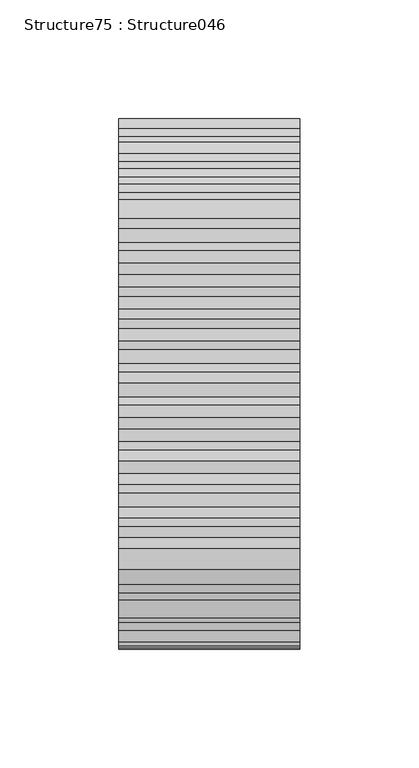
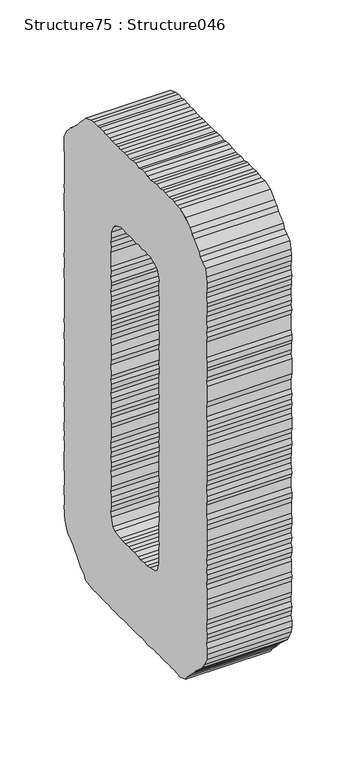
"""IFC4 building model written with IfcOpenShell, lengths in millimetres: proxy geometry, Structure75 : Structure046."""

from ifc_helpers import new_model, si_unit, frame, origin, place, context, project, spatial, polyline, outline, extrude, source, transform, mapped, element, save


def structure75_structure046_599be4c7(model_context):
    return source(origin(), model_context, "Body", "SweptSolid", [
        extrude(outline(polyline([(278111.8907934, 3554.0087015), (278103.1103976, 3552.242032), (278099.0090285, 3551.6675836), (278094.9092641, 3552.242032), (278090.2286327, 3552.242032), (278084.9478793, 3551.6675836), (278080.267248, 3551.6675836), (278076.1658789, 3552.242032), (278070.8851255, 3551.0658569), (278065.625232, 3551.6675836), (278061.5013985, 3551.0658569), (278057.401634, 3551.0658569), (278052.7210027, 3552.242032), (278048.0195115, 3552.242032), (278043.3613446, 3551.6675836), (278029.2761264, 3551.6675836), (278024.0162328, 3552.242032), (278019.9164683, 3552.242032), (278015.2133726, 3551.0658569), (278010.5343459, 3551.0658569), (278006.4329768, 3552.242032), (278001.1506188, 3551.6675836), (277997.652581, 3552.242032), (277991.7909607, 3551.6675836), (277987.6687318, 3551.6675836), (277982.4088383, 3552.242032), (277978.3074692, 3551.6675836), (277974.2077047, 3552.242032), (277969.5270734, 3551.6675836), (277964.2447154, 3551.0658569), (277956.0435818, 3554.0087015), (277953.1248062, 3558.1100706), (277946.6614593, 3564.54293), (277943.7426837, 3568.0682461), (277939.6413146, 3572.1423369), (277936.1208124, 3575.0851816), (277933.2004322, 3578.0103756), (277929.6799299, 3580.9532202), (277926.7595497, 3585.6274331), (277923.2390475, 3592.6700423), (277922.6373208, 3597.9540049), (277922.6373208, 3603.2122938), (277923.8183097, 3607.8961343), (277923.2390475, 3612.5976255), (277922.6373208, 3616.69739), (277923.8183097, 3621.3732075), (277923.8183097, 3625.472972), (277923.2390475, 3630.1824862), (277923.2390475, 3640.7167147), (277922.6373208, 3645.4262289), (277923.2390475, 3649.5003197), (277923.2390475, 3659.4584952), (277923.8183097, 3663.5598643), (277922.6373208, 3668.8261762), (277922.6373208, 3673.5276674), (277923.8183097, 3677.0449605), (277922.6373208, 3682.3289231), (277923.8183097, 3686.4030139), (277923.2390475, 3691.6869765), (277922.6373208, 3696.3884676), (277922.6373208, 3701.0723082), (277923.2390475, 3705.1720727), (277923.2390475, 3715.7143242), (277922.6373208, 3720.9726131), (277922.6373208, 3725.0996559), (277923.8183097, 3730.3563402), (277923.8183097, 3739.1592005), (277922.6373208, 3743.2332913), (277923.2390475, 3747.9428055), (277923.8183097, 3753.2171405), (277923.8183097, 3757.8753073), (277923.2390475, 3762.5848215), (277923.2390475, 3767.2590344), (277922.6373208, 3771.3860772), (277923.2390475, 3777.2444882), (277923.2390475, 3781.9299333), (277922.6373208, 3786.6298199), (277922.6373208, 3795.960595), (277923.2390475, 3800.6717138), (277923.2390475, 3805.3459267), (277922.6373208, 3810.0474179), (277923.2390475, 3813.5743386), (277922.6373208, 3819.4150989), (277923.8183097, 3823.5341187), (277923.8183097, 3832.3161191), (277922.6373208, 3838.1761347), (277922.6373208, 3852.8181507), (277923.8183097, 3856.9179152), (277923.2390475, 3861.0192843), (277923.2390475, 3866.8776953), (277922.6373208, 3870.4030114), (277922.6373208, 3875.686974), (277923.8183097, 3879.7610648), (277923.8183097, 3894.4030808), (277922.6373208, 3899.1061766), (277923.8183097, 3903.2059411), (277923.2390475, 3907.888177), (277923.8183097, 3913.1641166), (277923.8183097, 3918.4480792), (277923.2390475, 3923.1319197), (277923.2390475, 3927.8077372), (277922.6373208, 3931.9058971), (277923.8183097, 3936.6186205), (277923.8183097, 3940.718385), (277923.2390475, 3945.4182716), (277923.2390475, 3950.6765605), (277923.8183097, 3955.9348494), (277925.5785608, 3962.9774586), (277930.2591922, 3966.5043792), (277933.7796944, 3969.418341), (277935.5399455, 3973.5197101), (277943.140957, 3980.5623192), (277946.0821971, 3984.0635662), (277949.6026993, 3987.5792547), (277956.0435818, 3993.4472933), (277964.8239776, 3996.390138), (277969.5270734, 3996.390138), (277974.2077047, 3997.5486624), (277977.7282069, 3997.5486624), (277982.4088383, 3996.9645864), (277988.2704585, 3997.5486624), (277991.7909607, 3997.5486624), (277996.4715921, 3996.390138), (278001.7523455, 3997.5486624), (278006.4329768, 3996.390138), (278009.9326192, 3996.390138), (278015.2133726, 3996.9645864), (278019.9164683, 3997.5486624), (278025.1763619, 3997.5486624), (278028.6968641, 3996.390138), (278034.5584844, 3997.5486624), (278039.2375111, 3996.9645864), (278042.7596179, 3996.390138), (278048.6212382, 3996.390138), (278052.1417404, 3996.9645864), (278057.401634, 3996.390138), (278061.5013985, 3996.9645864), (278065.625232, 3996.390138), (278070.8851255, 3996.390138), (278074.98489, 3996.9645864), (278080.267248, 3996.9645864), (278084.9478793, 3997.5486624), (278090.2286327, 3997.5486624), (278093.7282751, 3996.9645864), (278099.5898954, 3996.9645864), (278103.6896599, 3996.390138), (278111.8907934, 3993.4472933), (278114.8336381, 3989.9460463), (278118.3541403, 3986.4046842), (278121.2729159, 3983.4794902), (278124.7950228, 3979.3781211), (278127.7137984, 3976.4368811), (278131.2359052, 3973.5197101), (278135.9149319, 3969.994394), (278138.2560499, 3967.0788276), (278141.7765522, 3962.9774586), (278145.8779213, 3955.360401), (278145.8779213, 3946.5511223), (278144.6969323, 3936.0345445), (278145.298659, 3931.3346579), (278145.298659, 3927.2332888), (278144.6969323, 3921.9733953), (278145.298659, 3917.8479571), (278144.6969323, 3912.5896682), (278145.8779213, 3908.46423), (278145.298659, 3904.3901392), (278145.8779213, 3899.7046941), (278145.8779213, 3889.1463965), (278144.6969323, 3880.9452629), (278144.6969323, 3876.263027), (278145.298659, 3871.5599312), (278144.6969323, 3866.3032469), (278144.6969323, 3847.5598618), (278145.8779213, 3843.432819), (278144.6969323, 3837.6000817), (278145.298659, 3832.3161191), (278145.8779213, 3828.790803), (278145.8779213, 3823.5341187), (278144.6969323, 3818.8310229), (278144.6969323, 3795.4037973), (278145.298659, 3790.7039107), (278144.6969323, 3785.4456218), (278145.8779213, 3780.7441306), (278144.6969323, 3776.6427615), (278145.298659, 3771.3860772), (278145.8779213, 3767.8607611), (278144.6969323, 3758.485057), (278144.6969323, 3752.6170184), (278145.298659, 3749.117376), (278144.6969323, 3743.8414364), (278145.8779213, 3739.7416719), (278144.6969323, 3734.47536), (278144.6969323, 3730.3563402), (278145.298659, 3725.0996559), (278145.8779213, 3720.9726131), (278145.298659, 3715.7143242), (278145.298659, 3705.7545441), (278145.8779213, 3700.4705815), (278144.6969323, 3696.3884676), (278144.6969323, 3691.6869765), (278145.298659, 3686.4030139), (278145.8779213, 3682.3289231), (278145.8779213, 3677.6274319), (278145.298659, 3672.3691429), (278145.8779213, 3668.8261762), (278145.298659, 3663.5598643), (278145.298659, 3658.3015753), (278145.8779213, 3653.6000842), (278145.8779213, 3640.114988), (278145.298659, 3635.4407751), (278144.6969323, 3631.3410106), (278144.6969323, 3626.6571701), (278145.8779213, 3621.9813526), (278145.8779213, 3617.2718384), (278144.6969323, 3611.4134274), (278145.298659, 3606.7295868), (278145.8779213, 3603.2122938), (278145.298659, 3597.9540049), (278144.6969323, 3593.8285667), (278141.7765522, 3585.0706354), (278139.4370388, 3580.9532202), (278134.7564075, 3578.0103756), (278131.2359052, 3574.5107332), (278128.3155251, 3572.1423369), (278124.7950228, 3567.4857747), (278118.9334026, 3561.025637), (278114.2527713, 3558.1100706), (278111.8907934, 3554.0087015)]), holes=[polyline([(278003.4917367, 3918.4480792), (278001.1506188, 3916.6653636), (277997.652581, 3908.46423), (277998.8111054, 3903.7884125), (277998.8111054, 3895.5888836), (277997.652581, 3890.320967), (277997.652581, 3880.9452629), (277998.8111054, 3875.686974), (277998.2318432, 3870.9790644), (277998.2318432, 3861.6178018), (277997.652581, 3858.1021133), (277997.652581, 3848.7167816), (277998.8111054, 3843.432819), (277997.652581, 3838.1761347), (277997.652581, 3833.4730389), (277998.8111054, 3828.790803), (277997.652581, 3824.7167122), (277997.652581, 3820.5896694), (277998.8111054, 3815.3313805), (277998.2318432, 3811.2043377), (277998.2318432, 3802.448011), (277997.652581, 3797.1463977), (277998.2318432, 3792.4705802), (277998.2318432, 3787.7867397), (277998.8111054, 3783.0868532), (277998.2318432, 3777.8285642), (277998.8111054, 3774.3032481), (277998.8111054, 3769.6274306), (277997.652581, 3764.9435901), (277997.652581, 3759.0595054), (277998.8111054, 3754.3756649), (277997.652581, 3749.701452), (277997.652581, 3746.1745313), (277998.8111054, 3740.9162424), (277998.2318432, 3736.7988273), (277998.8111054, 3730.9323932), (277998.8111054, 3726.8566978), (277998.2318432, 3722.7312597), (277997.652581, 3717.4729707), (277998.8111054, 3712.7971532), (277998.2318432, 3708.087639), (277998.2318432, 3704.5879966), (277997.652581, 3699.3136616), (277997.652581, 3695.2122926), (277998.2318432, 3690.512406), (277997.652581, 3685.8285655), (277997.652581, 3681.1447249), (277998.8111054, 3675.2863139), (277998.8111054, 3671.1849448), (277998.2318432, 3666.5027089), (277998.2318432, 3662.3836892), (277997.652581, 3657.1254002), (277998.8111054, 3652.4431643), (277998.8111054, 3648.3161216), (277998.2318432, 3643.0578326), (277998.2318432, 3638.9580681), (278001.1506188, 3630.7392839), (278003.4917367, 3628.4158166), (278011.1136081, 3626.6571701), (278016.3943615, 3625.472972), (278020.4957306, 3626.0554434), (278026.3573508, 3625.472972), (278029.8778531, 3626.0554434), (278035.7394733, 3626.6571701), (278040.4201046, 3626.0554434), (278044.5198691, 3626.6571701), (278049.8022271, 3626.0554434), (278053.9019916, 3626.0554434), (278058.0033607, 3626.6571701), (278066.1820298, 3628.4158166), (278069.1232698, 3630.7392839), (278072.0661145, 3637.7995437), (278072.6453767, 3643.0578326), (278071.4643878, 3648.3161216), (278072.0661145, 3651.8590883), (278072.0661145, 3657.1254002), (278072.6453767, 3662.3836892), (278072.0661145, 3667.0851803), (278072.0661145, 3675.8687854), (278072.6453767, 3681.1447249), (278071.4643878, 3685.8285655), (278072.0661145, 3689.9540036), (278072.6453767, 3694.6298211), (278072.0661145, 3699.8881101), (278072.6453767, 3703.4134261), (278072.6453767, 3708.6717151), (278072.0661145, 3713.3555556), (278072.0661145, 3723.3313817), (278071.4643878, 3726.8566978), (278072.6453767, 3732.1149867), (278071.4643878, 3736.7988273), (278072.0661145, 3740.3161203), (278072.0661145, 3746.1745313), (278071.4643878, 3750.8583719), (278072.6453767, 3755.559863), (278072.0661145, 3759.6596275), (278071.4643878, 3764.9435901), (278072.6453767, 3768.4432325), (278071.4643878, 3773.11905), (278072.6453767, 3782.5027771), (278071.4643878, 3787.7867397), (278072.0661145, 3792.4705802), (278072.0661145, 3801.2718359), (278072.6453767, 3806.5317294), (278071.4643878, 3811.7884138), (278072.0661145, 3816.4883003), (278071.4643878, 3820.5896694), (278072.0661145, 3824.1149855), (278071.4643878, 3828.790803), (278072.6453767, 3834.0474873), (278072.6453767, 3838.1761347), (278071.4643878, 3844.0345457), (278071.4643878, 3848.1166595), (278072.6453767, 3852.2340747), (278072.0661145, 3858.1021133), (278071.4643878, 3861.6178018), (278072.6453767, 3866.3032469), (278071.4643878, 3872.1440073), (278072.6453767, 3875.686974), (278072.6453767, 3889.7208449), (278072.0661145, 3895.0048075), (278072.6453767, 3899.1061766), (278071.4643878, 3903.7884125), (278071.4643878, 3909.6468235), (278068.5440076, 3916.0909152), (278066.1820298, 3919.0321552), (278058.0033607, 3922.5494483), (278053.3002649, 3922.5494483), (278049.2005004, 3921.9733953), (278043.9181424, 3922.5494483), (278039.2375111, 3922.5494483), (278034.5584844, 3921.3748778), (278029.8778531, 3922.5494483), (278025.1763619, 3921.3748778), (278020.4957306, 3922.5494483), (278016.3943615, 3921.9733953), (278011.7153348, 3922.5494483), (278003.4917367, 3918.4480792)])]), frame((-59031.6926606, 0.0, 0.0), z_axis=(1.0, 0.0, 0.0), x_axis=(0.0, 1.0, 0.0)), (0.0, 0.0, 1.0), 76.2),
    ])


if __name__ == "__main__":
    model = new_model("IFC4")
    model_context = context("Model", 3, world=origin())
    ifc_project = project(units=[si_unit("LENGTHUNIT", "METRE", prefix="MILLI")], contexts=[model_context])
    site = spatial("IfcSite", under=ifc_project)
    building = spatial("IfcBuilding", under=site)
    placement = place(None, origin())
    structure75_structure046_shape = structure75_structure046_599be4c7(model_context)
    element("IfcBuildingElementProxy", 1, Name="Structure75 : Structure046", ObjectType="Structure75 : Structure046", at=placement, inside=building, context=model_context, shape_type="MappedRepresentation", body=[
        mapped(structure75_structure046_shape, transform((0.0, 0.0, 0.0), x_axis=(1.0, 0.0, 0.0), y_axis=(0.0, 1.0, 0.0), z_axis=(0.0, 0.0, 1.0))),
    ])
    save(model, "model.ifc")

# Revit data of these elements
# Type "Structure75 : Structure046"
#   NameOverride = "Structure046"
# Element 1 (IfcBuildingElementProxy, "Structure75 : Structure046")
#   Materials on its faces: "BRUSHED ALUM. LETTERING"
# Materials
#   "BRUSHED ALUM. LETTERING": class "Unassigned", colour RGB 169 181 186, transparency 0, Cost = 0
